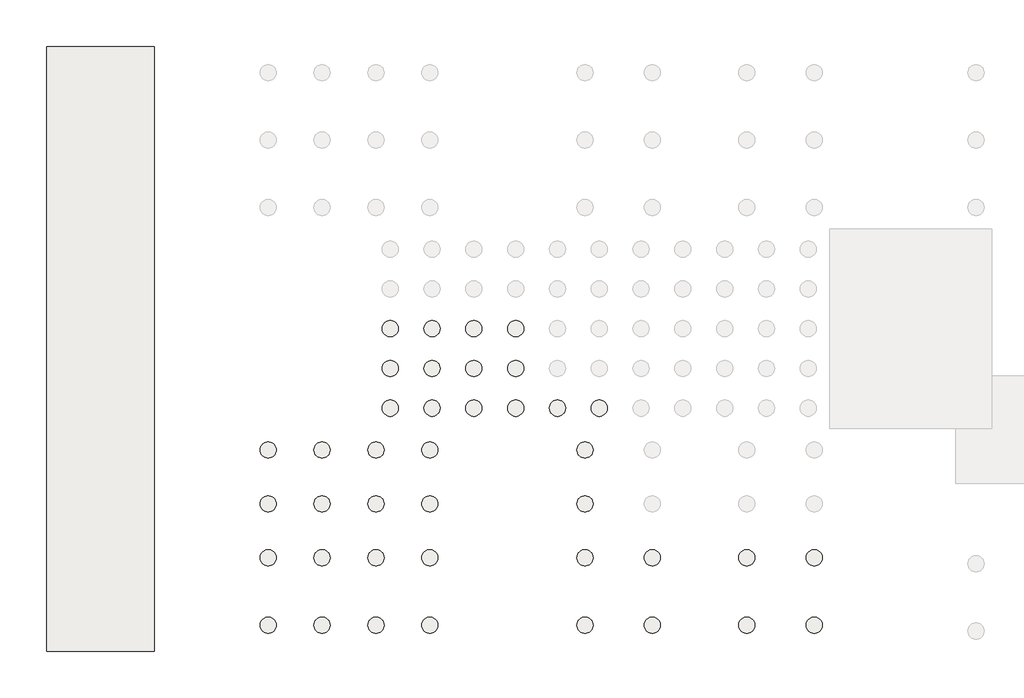
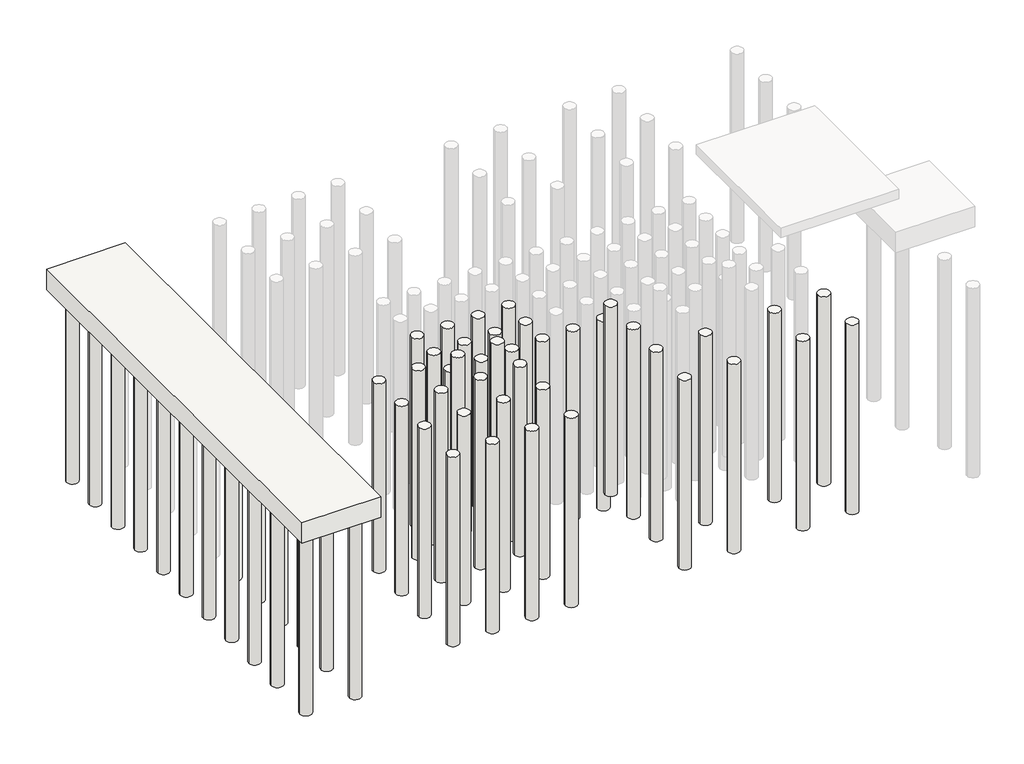
# One storey, part 1 of 3: 58 slabs.
"""IFC4 building model written with IfcOpenShell, lengths in millimetres."""

from ifc_helpers import new_model, si_unit, point, frame, frame_2d, origin, place, context, project, spatial, polyline, circle_curve, trimmed, segment, composite_curve, outline, extrude, element, save

model = new_model("IFC4")

# Units and contexts
model_context = context("Model", 3, world=origin())
ifc_project = project(units=[si_unit("LENGTHUNIT", "METRE", prefix="MILLI")], contexts=[model_context])

# Site, building, storey
site = spatial("IfcSite", under=ifc_project)
building = spatial("IfcBuilding", under=site)
storey = spatial("IfcBuildingStorey", under=building, Name="B.O.F(FDN)", Elevation=-2500.0279945)

# Slabs
placement = place(None, origin())
element("IfcSlab", 1, ObjectType="Foundation Rectangular(Non-Pile) : H_SF_ACF_W4000xL22440xT1100_Protection", at=placement, inside=storey, context=model_context, shape_type="SweptSolid", body=[
    extrude(outline(polyline([(1785.0, 41219.5208589), (1785.0, 18779.5208589), (-2215.0, 18779.5208589), (-2215.0, 41219.5208589), (1785.0, 41219.5208589)])), frame((0.0, 0.0, -3600.0279945), z_axis=(0.0, 0.0, 1.0), x_axis=(1.0, 0.0, 0.0)), (0.0, 0.0, 1.0), 1100.0),
])
element("IfcSlab", 2, ObjectType="Pile : H_SF_API_Steel Pile D508x12t_L10m", at=placement, inside=storey, context=model_context, shape_type="SweptSolid", body=[
    extrude(outline(composite_curve([segment(trimmed(circle_curve(frame_2d((-1465.0, 40249.5208589)), 300.0), [point((-1765.0, 40249.5208589))], [point((-1165.0, 40249.5208589))], False, "CARTESIAN"), True, "CONTINUOUS"), segment(trimmed(circle_curve(frame_2d((-1465.0, 40249.5208589)), 300.0), [point((-1165.0, 40249.5208589))], [point((-1765.0, 40249.5208589))], False, "CARTESIAN"), True, "CONTINUOUS")], self_intersect=False)), frame((0.0, 0.0, -13500.0279945), z_axis=(0.0, 0.0, 1.0), x_axis=(1.0, 0.0, 0.0)), (0.0, 0.0, 1.0), 10150.0),
])
element("IfcSlab", 3, ObjectType="Pile : H_SF_API_Steel Pile D508x12t_L10m", at=placement, inside=storey, context=model_context, shape_type="SweptSolid", body=[
    extrude(outline(composite_curve([segment(trimmed(circle_curve(frame_2d((-1465.0, 19749.5208589)), 300.0), [point((-1765.0, 19749.5208589))], [point((-1165.0, 19749.5208589))], False, "CARTESIAN"), True, "CONTINUOUS"), segment(trimmed(circle_curve(frame_2d((-1465.0, 19749.5208589)), 300.0), [point((-1165.0, 19749.5208589))], [point((-1765.0, 19749.5208589))], False, "CARTESIAN"), True, "CONTINUOUS")], self_intersect=False)), frame((0.0, 0.0, -13500.0279945), z_axis=(0.0, 0.0, 1.0), x_axis=(1.0, 0.0, 0.0)), (0.0, 0.0, 1.0), 10150.0),
])
element("IfcSlab", 4, ObjectType="Pile : H_SF_API_Steel Pile D508x12t_L10m", at=placement, inside=storey, context=model_context, shape_type="SweptSolid", body=[
    extrude(outline(composite_curve([segment(trimmed(circle_curve(frame_2d((1035.0, 19749.5208589)), 300.0), [point((1335.0, 19749.5208589))], [point((735.0, 19749.5208589))], False, "CARTESIAN"), True, "CONTINUOUS"), segment(trimmed(circle_curve(frame_2d((1035.0, 19749.5208589)), 300.0), [point((735.0, 19749.5208589))], [point((1335.0, 19749.5208589))], False, "CARTESIAN"), True, "CONTINUOUS")], self_intersect=False)), frame((0.0, 0.0, -13500.0279945), z_axis=(0.0, 0.0, 1.0), x_axis=(1.0, 0.0, 0.0)), (0.0, 0.0, 1.0), 10150.0),
])
element("IfcSlab", 5, ObjectType="Pile : H_SF_API_Steel Pile D508x12t_L10m", at=placement, inside=storey, context=model_context, shape_type="SweptSolid", body=[
    extrude(outline(composite_curve([segment(trimmed(circle_curve(frame_2d((-1465.0, 38249.5208589)), 300.0), [point((-1765.0, 38249.5208589))], [point((-1165.0, 38249.5208589))], False, "CARTESIAN"), True, "CONTINUOUS"), segment(trimmed(circle_curve(frame_2d((-1465.0, 38249.5208589)), 300.0), [point((-1165.0, 38249.5208589))], [point((-1765.0, 38249.5208589))], False, "CARTESIAN"), True, "CONTINUOUS")], self_intersect=False)), frame((0.0, 0.0, -13500.0279945), z_axis=(0.0, 0.0, 1.0), x_axis=(1.0, 0.0, 0.0)), (0.0, 0.0, 1.0), 10150.0),
])
element("IfcSlab", 6, ObjectType="Pile : H_SF_API_Steel Pile D508x12t_L10m", at=placement, inside=storey, context=model_context, shape_type="SweptSolid", body=[
    extrude(outline(composite_curve([segment(trimmed(circle_curve(frame_2d((-1465.0, 36249.5208589)), 300.0), [point((-1765.0, 36249.5208589))], [point((-1165.0, 36249.5208589))], False, "CARTESIAN"), True, "CONTINUOUS"), segment(trimmed(circle_curve(frame_2d((-1465.0, 36249.5208589)), 300.0), [point((-1165.0, 36249.5208589))], [point((-1765.0, 36249.5208589))], False, "CARTESIAN"), True, "CONTINUOUS")], self_intersect=False)), frame((0.0, 0.0, -13500.0279945), z_axis=(0.0, 0.0, 1.0), x_axis=(1.0, 0.0, 0.0)), (0.0, 0.0, 1.0), 10150.0),
])
element("IfcSlab", 7, ObjectType="Pile : H_SF_API_Steel Pile D508x12t_L10m", at=placement, inside=storey, context=model_context, shape_type="SweptSolid", body=[
    extrude(outline(composite_curve([segment(trimmed(circle_curve(frame_2d((-1465.0, 34249.5208589)), 300.0), [point((-1765.0, 34249.5208589))], [point((-1165.0, 34249.5208589))], False, "CARTESIAN"), True, "CONTINUOUS"), segment(trimmed(circle_curve(frame_2d((-1465.0, 34249.5208589)), 300.0), [point((-1165.0, 34249.5208589))], [point((-1765.0, 34249.5208589))], False, "CARTESIAN"), True, "CONTINUOUS")], self_intersect=False)), frame((0.0, 0.0, -13500.0279945), z_axis=(0.0, 0.0, 1.0), x_axis=(1.0, 0.0, 0.0)), (0.0, 0.0, 1.0), 10150.0),
])
element("IfcSlab", 8, ObjectType="Pile : H_SF_API_Steel Pile D508x12t_L10m", at=placement, inside=storey, context=model_context, shape_type="SweptSolid", body=[
    extrude(outline(composite_curve([segment(trimmed(circle_curve(frame_2d((-1465.0, 32249.5208589)), 300.0), [point((-1765.0, 32249.5208589))], [point((-1165.0, 32249.5208589))], False, "CARTESIAN"), True, "CONTINUOUS"), segment(trimmed(circle_curve(frame_2d((-1465.0, 32249.5208589)), 300.0), [point((-1165.0, 32249.5208589))], [point((-1765.0, 32249.5208589))], False, "CARTESIAN"), True, "CONTINUOUS")], self_intersect=False)), frame((0.0, 0.0, -13500.0279945), z_axis=(0.0, 0.0, 1.0), x_axis=(1.0, 0.0, 0.0)), (0.0, 0.0, 1.0), 10150.0),
])
element("IfcSlab", 9, ObjectType="Pile : H_SF_API_Steel Pile D508x12t_L10m", at=placement, inside=storey, context=model_context, shape_type="SweptSolid", body=[
    extrude(outline(composite_curve([segment(trimmed(circle_curve(frame_2d((-1465.0, 30249.5208589)), 300.0), [point((-1765.0, 30249.5208589))], [point((-1165.0, 30249.5208589))], False, "CARTESIAN"), True, "CONTINUOUS"), segment(trimmed(circle_curve(frame_2d((-1465.0, 30249.5208589)), 300.0), [point((-1165.0, 30249.5208589))], [point((-1765.0, 30249.5208589))], False, "CARTESIAN"), True, "CONTINUOUS")], self_intersect=False)), frame((0.0, 0.0, -13500.0279945), z_axis=(0.0, 0.0, 1.0), x_axis=(1.0, 0.0, 0.0)), (0.0, 0.0, 1.0), 10150.0),
])
element("IfcSlab", 10, ObjectType="Pile : H_SF_API_Steel Pile D508x12t_L10m", at=placement, inside=storey, context=model_context, shape_type="SweptSolid", body=[
    extrude(outline(composite_curve([segment(trimmed(circle_curve(frame_2d((1035.0, 30249.5208589)), 300.0), [point((1335.0, 30249.5208589))], [point((735.0, 30249.5208589))], False, "CARTESIAN"), True, "CONTINUOUS"), segment(trimmed(circle_curve(frame_2d((1035.0, 30249.5208589)), 300.0), [point((735.0, 30249.5208589))], [point((1335.0, 30249.5208589))], False, "CARTESIAN"), True, "CONTINUOUS")], self_intersect=False)), frame((0.0, 0.0, -13500.0279945), z_axis=(0.0, 0.0, 1.0), x_axis=(1.0, 0.0, 0.0)), (0.0, 0.0, 1.0), 10150.0),
])
element("IfcSlab", 11, ObjectType="Pile : H_SF_API_Steel Pile D508x12t_L10m", at=placement, inside=storey, context=model_context, shape_type="SweptSolid", body=[
    extrude(outline(composite_curve([segment(trimmed(circle_curve(frame_2d((-1465.0, 28249.5208589)), 300.0), [point((-1765.0, 28249.5208589))], [point((-1165.0, 28249.5208589))], False, "CARTESIAN"), True, "CONTINUOUS"), segment(trimmed(circle_curve(frame_2d((-1465.0, 28249.5208589)), 300.0), [point((-1165.0, 28249.5208589))], [point((-1765.0, 28249.5208589))], False, "CARTESIAN"), True, "CONTINUOUS")], self_intersect=False)), frame((0.0, 0.0, -13500.0279945), z_axis=(0.0, 0.0, 1.0), x_axis=(1.0, 0.0, 0.0)), (0.0, 0.0, 1.0), 10150.0),
])
element("IfcSlab", 12, ObjectType="Pile : H_SF_API_Steel Pile D508x12t_L10m", at=placement, inside=storey, context=model_context, shape_type="SweptSolid", body=[
    extrude(outline(composite_curve([segment(trimmed(circle_curve(frame_2d((1035.0, 28249.5208589)), 300.0), [point((1335.0, 28249.5208589))], [point((735.0, 28249.5208589))], False, "CARTESIAN"), True, "CONTINUOUS"), segment(trimmed(circle_curve(frame_2d((1035.0, 28249.5208589)), 300.0), [point((735.0, 28249.5208589))], [point((1335.0, 28249.5208589))], False, "CARTESIAN"), True, "CONTINUOUS")], self_intersect=False)), frame((0.0, 0.0, -13500.0279945), z_axis=(0.0, 0.0, 1.0), x_axis=(1.0, 0.0, 0.0)), (0.0, 0.0, 1.0), 10150.0),
])
element("IfcSlab", 13, ObjectType="Pile : H_SF_API_Steel Pile D508x12t_L10m", at=placement, inside=storey, context=model_context, shape_type="SweptSolid", body=[
    extrude(outline(composite_curve([segment(trimmed(circle_curve(frame_2d((-1465.0, 26249.5208589)), 300.0), [point((-1765.0, 26249.5208589))], [point((-1165.0, 26249.5208589))], False, "CARTESIAN"), True, "CONTINUOUS"), segment(trimmed(circle_curve(frame_2d((-1465.0, 26249.5208589)), 300.0), [point((-1165.0, 26249.5208589))], [point((-1765.0, 26249.5208589))], False, "CARTESIAN"), True, "CONTINUOUS")], self_intersect=False)), frame((0.0, 0.0, -13500.0279945), z_axis=(0.0, 0.0, 1.0), x_axis=(1.0, 0.0, 0.0)), (0.0, 0.0, 1.0), 10150.0),
])
element("IfcSlab", 14, ObjectType="Pile : H_SF_API_Steel Pile D508x12t_L10m", at=placement, inside=storey, context=model_context, shape_type="SweptSolid", body=[
    extrude(outline(composite_curve([segment(trimmed(circle_curve(frame_2d((1035.0, 26249.5208589)), 300.0), [point((1335.0, 26249.5208589))], [point((735.0, 26249.5208589))], False, "CARTESIAN"), True, "CONTINUOUS"), segment(trimmed(circle_curve(frame_2d((1035.0, 26249.5208589)), 300.0), [point((735.0, 26249.5208589))], [point((1335.0, 26249.5208589))], False, "CARTESIAN"), True, "CONTINUOUS")], self_intersect=False)), frame((0.0, 0.0, -13500.0279945), z_axis=(0.0, 0.0, 1.0), x_axis=(1.0, 0.0, 0.0)), (0.0, 0.0, 1.0), 10150.0),
])
element("IfcSlab", 15, ObjectType="Pile : H_SF_API_Steel Pile D508x12t_L10m", at=placement, inside=storey, context=model_context, shape_type="SweptSolid", body=[
    extrude(outline(composite_curve([segment(trimmed(circle_curve(frame_2d((-1465.0, 24249.5208589)), 300.0), [point((-1765.0, 24249.5208589))], [point((-1165.0, 24249.5208589))], False, "CARTESIAN"), True, "CONTINUOUS"), segment(trimmed(circle_curve(frame_2d((-1465.0, 24249.5208589)), 300.0), [point((-1165.0, 24249.5208589))], [point((-1765.0, 24249.5208589))], False, "CARTESIAN"), True, "CONTINUOUS")], self_intersect=False)), frame((0.0, 0.0, -13500.0279945), z_axis=(0.0, 0.0, 1.0), x_axis=(1.0, 0.0, 0.0)), (0.0, 0.0, 1.0), 10150.0),
])
element("IfcSlab", 16, ObjectType="Pile : H_SF_API_Steel Pile D508x12t_L10m", at=placement, inside=storey, context=model_context, shape_type="SweptSolid", body=[
    extrude(outline(composite_curve([segment(trimmed(circle_curve(frame_2d((1035.0, 24249.5208589)), 300.0), [point((1335.0, 24249.5208589))], [point((735.0, 24249.5208589))], False, "CARTESIAN"), True, "CONTINUOUS"), segment(trimmed(circle_curve(frame_2d((1035.0, 24249.5208589)), 300.0), [point((735.0, 24249.5208589))], [point((1335.0, 24249.5208589))], False, "CARTESIAN"), True, "CONTINUOUS")], self_intersect=False)), frame((0.0, 0.0, -13500.0279945), z_axis=(0.0, 0.0, 1.0), x_axis=(1.0, 0.0, 0.0)), (0.0, 0.0, 1.0), 10150.0),
])
element("IfcSlab", 17, ObjectType="Pile : H_SF_API_Steel Pile D508x12t_L10m", at=placement, inside=storey, context=model_context, shape_type="SweptSolid", body=[
    extrude(outline(composite_curve([segment(trimmed(circle_curve(frame_2d((-1465.0, 22249.5208589)), 300.0), [point((-1765.0, 22249.5208589))], [point((-1165.0, 22249.5208589))], False, "CARTESIAN"), True, "CONTINUOUS"), segment(trimmed(circle_curve(frame_2d((-1465.0, 22249.5208589)), 300.0), [point((-1165.0, 22249.5208589))], [point((-1765.0, 22249.5208589))], False, "CARTESIAN"), True, "CONTINUOUS")], self_intersect=False)), frame((0.0, 0.0, -13500.0279945), z_axis=(0.0, 0.0, 1.0), x_axis=(1.0, 0.0, 0.0)), (0.0, 0.0, 1.0), 10150.0),
])
element("IfcSlab", 18, ObjectType="Pile : H_SF_API_Steel Pile D508x12t_L10m", at=placement, inside=storey, context=model_context, shape_type="SweptSolid", body=[
    extrude(outline(composite_curve([segment(trimmed(circle_curve(frame_2d((1035.0, 22249.5208589)), 300.0), [point((1335.0, 22249.5208589))], [point((735.0, 22249.5208589))], False, "CARTESIAN"), True, "CONTINUOUS"), segment(trimmed(circle_curve(frame_2d((1035.0, 22249.5208589)), 300.0), [point((735.0, 22249.5208589))], [point((1335.0, 22249.5208589))], False, "CARTESIAN"), True, "CONTINUOUS")], self_intersect=False)), frame((0.0, 0.0, -13500.0279945), z_axis=(0.0, 0.0, 1.0), x_axis=(1.0, 0.0, 0.0)), (0.0, 0.0, 1.0), 10150.0),
])
element("IfcSlab", 19, ObjectType="Pile : H_SF_API_Steel Pile D508x12t_L10m", at=placement, inside=storey, context=model_context, shape_type="SweptSolid", body=[
    extrude(outline(composite_curve([segment(trimmed(circle_curve(frame_2d((8000.0, 19749.5208589)), 300.0), [point((8300.0, 19749.5208589))], [point((7700.0, 19749.5208589))], False, "CARTESIAN"), True, "CONTINUOUS"), segment(trimmed(circle_curve(frame_2d((8000.0, 19749.5208589)), 300.0), [point((7700.0, 19749.5208589))], [point((8300.0, 19749.5208589))], False, "CARTESIAN"), True, "CONTINUOUS")], self_intersect=False)), frame((0.0, 0.0, -12400.0279945), z_axis=(0.0, 0.0, 1.0), x_axis=(1.0, 0.0, 0.0)), (0.0, 0.0, 1.0), 10150.0),
])
element("IfcSlab", 20, ObjectType="Pile : H_SF_API_Steel Pile D508x12t_L10m", at=placement, inside=storey, context=model_context, shape_type="SweptSolid", body=[
    extrude(outline(composite_curve([segment(trimmed(circle_curve(frame_2d((6000.0, 19749.5208589)), 300.0), [point((5700.0, 19749.5208589))], [point((6300.0, 19749.5208589))], False, "CARTESIAN"), True, "CONTINUOUS"), segment(trimmed(circle_curve(frame_2d((6000.0, 19749.5208589)), 300.0), [point((6300.0, 19749.5208589))], [point((5700.0, 19749.5208589))], False, "CARTESIAN"), True, "CONTINUOUS")], self_intersect=False)), frame((0.0, 0.0, -12400.0279945), z_axis=(0.0, 0.0, 1.0), x_axis=(1.0, 0.0, 0.0)), (0.0, 0.0, 1.0), 10150.0),
])
element("IfcSlab", 21, ObjectType="Pile : H_SF_API_Steel Pile D508x12t_L10m", at=placement, inside=storey, context=model_context, shape_type="SweptSolid", body=[
    extrude(outline(composite_curve([segment(trimmed(circle_curve(frame_2d((8000.0, 22249.5208589)), 300.0), [point((8300.0, 22249.5208589))], [point((7700.0, 22249.5208589))], False, "CARTESIAN"), True, "CONTINUOUS"), segment(trimmed(circle_curve(frame_2d((8000.0, 22249.5208589)), 300.0), [point((7700.0, 22249.5208589))], [point((8300.0, 22249.5208589))], False, "CARTESIAN"), True, "CONTINUOUS")], self_intersect=False)), frame((0.0, 0.0, -12400.0279945), z_axis=(0.0, 0.0, 1.0), x_axis=(1.0, 0.0, 0.0)), (0.0, 0.0, 1.0), 10150.0),
])
element("IfcSlab", 22, ObjectType="Pile : H_SF_API_Steel Pile D508x12t_L10m", at=placement, inside=storey, context=model_context, shape_type="SweptSolid", body=[
    extrude(outline(composite_curve([segment(trimmed(circle_curve(frame_2d((6000.0, 22249.5208589)), 300.0), [point((5700.0, 22249.5208589))], [point((6300.0, 22249.5208589))], False, "CARTESIAN"), True, "CONTINUOUS"), segment(trimmed(circle_curve(frame_2d((6000.0, 22249.5208589)), 300.0), [point((6300.0, 22249.5208589))], [point((5700.0, 22249.5208589))], False, "CARTESIAN"), True, "CONTINUOUS")], self_intersect=False)), frame((0.0, 0.0, -12400.0279945), z_axis=(0.0, 0.0, 1.0), x_axis=(1.0, 0.0, 0.0)), (0.0, 0.0, 1.0), 10150.0),
])
element("IfcSlab", 23, ObjectType="Pile : H_SF_API_Steel Pile D508x12t_L10m", at=placement, inside=storey, context=model_context, shape_type="SweptSolid", body=[
    extrude(outline(composite_curve([segment(trimmed(circle_curve(frame_2d((8000.0, 24249.5208589)), 300.0), [point((8300.0, 24249.5208589))], [point((7700.0, 24249.5208589))], False, "CARTESIAN"), True, "CONTINUOUS"), segment(trimmed(circle_curve(frame_2d((8000.0, 24249.5208589)), 300.0), [point((7700.0, 24249.5208589))], [point((8300.0, 24249.5208589))], False, "CARTESIAN"), True, "CONTINUOUS")], self_intersect=False)), frame((0.0, 0.0, -12400.0279945), z_axis=(0.0, 0.0, 1.0), x_axis=(1.0, 0.0, 0.0)), (0.0, 0.0, 1.0), 10150.0),
])
element("IfcSlab", 24, ObjectType="Pile : H_SF_API_Steel Pile D508x12t_L10m", at=placement, inside=storey, context=model_context, shape_type="SweptSolid", body=[
    extrude(outline(composite_curve([segment(trimmed(circle_curve(frame_2d((6000.0, 24249.5208589)), 300.0), [point((5700.0, 24249.5208589))], [point((6300.0, 24249.5208589))], False, "CARTESIAN"), True, "CONTINUOUS"), segment(trimmed(circle_curve(frame_2d((6000.0, 24249.5208589)), 300.0), [point((6300.0, 24249.5208589))], [point((5700.0, 24249.5208589))], False, "CARTESIAN"), True, "CONTINUOUS")], self_intersect=False)), frame((0.0, 0.0, -12400.0279945), z_axis=(0.0, 0.0, 1.0), x_axis=(1.0, 0.0, 0.0)), (0.0, 0.0, 1.0), 10150.0),
])
element("IfcSlab", 25, ObjectType="Pile : H_SF_API_Steel Pile D508x12t_L10m", at=placement, inside=storey, context=model_context, shape_type="SweptSolid", body=[
    extrude(outline(composite_curve([segment(trimmed(circle_curve(frame_2d((8000.0, 26249.5208589)), 300.0), [point((8300.0, 26249.5208589))], [point((7700.0, 26249.5208589))], False, "CARTESIAN"), True, "CONTINUOUS"), segment(trimmed(circle_curve(frame_2d((8000.0, 26249.5208589)), 300.0), [point((7700.0, 26249.5208589))], [point((8300.0, 26249.5208589))], False, "CARTESIAN"), True, "CONTINUOUS")], self_intersect=False)), frame((0.0, 0.0, -12400.0279945), z_axis=(0.0, 0.0, 1.0), x_axis=(1.0, 0.0, 0.0)), (0.0, 0.0, 1.0), 10150.0),
])
element("IfcSlab", 26, ObjectType="Pile : H_SF_API_Steel Pile D508x12t_L10m", at=placement, inside=storey, context=model_context, shape_type="SweptSolid", body=[
    extrude(outline(composite_curve([segment(trimmed(circle_curve(frame_2d((6000.0, 26249.5208589)), 300.0), [point((5700.0, 26249.5208589))], [point((6300.0, 26249.5208589))], False, "CARTESIAN"), True, "CONTINUOUS"), segment(trimmed(circle_curve(frame_2d((6000.0, 26249.5208589)), 300.0), [point((6300.0, 26249.5208589))], [point((5700.0, 26249.5208589))], False, "CARTESIAN"), True, "CONTINUOUS")], self_intersect=False)), frame((0.0, 0.0, -12400.0279945), z_axis=(0.0, 0.0, 1.0), x_axis=(1.0, 0.0, 0.0)), (0.0, 0.0, 1.0), 10150.0),
])
element("IfcSlab", 27, ObjectType="Pile : H_SF_API_Steel Pile D508x12t_L10m", at=placement, inside=storey, context=model_context, shape_type="SweptSolid", body=[
    extrude(outline(composite_curve([segment(trimmed(circle_curve(frame_2d((12000.0, 19749.5208589)), 300.0), [point((12300.0, 19749.5208589))], [point((11700.0, 19749.5208589))], False, "CARTESIAN"), True, "CONTINUOUS"), segment(trimmed(circle_curve(frame_2d((12000.0, 19749.5208589)), 300.0), [point((11700.0, 19749.5208589))], [point((12300.0, 19749.5208589))], False, "CARTESIAN"), True, "CONTINUOUS")], self_intersect=False)), frame((0.0, 0.0, -12400.0279945), z_axis=(0.0, 0.0, 1.0), x_axis=(1.0, 0.0, 0.0)), (0.0, 0.0, 1.0), 10150.0),
])
element("IfcSlab", 28, ObjectType="Pile : H_SF_API_Steel Pile D508x12t_L10m", at=placement, inside=storey, context=model_context, shape_type="SweptSolid", body=[
    extrude(outline(composite_curve([segment(trimmed(circle_curve(frame_2d((10000.0, 19749.5208589)), 300.0), [point((9700.0, 19749.5208589))], [point((10300.0, 19749.5208589))], False, "CARTESIAN"), True, "CONTINUOUS"), segment(trimmed(circle_curve(frame_2d((10000.0, 19749.5208589)), 300.0), [point((10300.0, 19749.5208589))], [point((9700.0, 19749.5208589))], False, "CARTESIAN"), True, "CONTINUOUS")], self_intersect=False)), frame((0.0, 0.0, -12400.0279945), z_axis=(0.0, 0.0, 1.0), x_axis=(1.0, 0.0, 0.0)), (0.0, 0.0, 1.0), 10150.0),
])
element("IfcSlab", 29, ObjectType="Pile : H_SF_API_Steel Pile D508x12t_L10m", at=placement, inside=storey, context=model_context, shape_type="SweptSolid", body=[
    extrude(outline(composite_curve([segment(trimmed(circle_curve(frame_2d((12000.0, 22249.5208589)), 300.0), [point((12300.0, 22249.5208589))], [point((11700.0, 22249.5208589))], False, "CARTESIAN"), True, "CONTINUOUS"), segment(trimmed(circle_curve(frame_2d((12000.0, 22249.5208589)), 300.0), [point((11700.0, 22249.5208589))], [point((12300.0, 22249.5208589))], False, "CARTESIAN"), True, "CONTINUOUS")], self_intersect=False)), frame((0.0, 0.0, -12400.0279945), z_axis=(0.0, 0.0, 1.0), x_axis=(1.0, 0.0, 0.0)), (0.0, 0.0, 1.0), 10150.0),
])
element("IfcSlab", 30, ObjectType="Pile : H_SF_API_Steel Pile D508x12t_L10m", at=placement, inside=storey, context=model_context, shape_type="SweptSolid", body=[
    extrude(outline(composite_curve([segment(trimmed(circle_curve(frame_2d((10000.0, 22249.5208589)), 300.0), [point((9700.0, 22249.5208589))], [point((10300.0, 22249.5208589))], False, "CARTESIAN"), True, "CONTINUOUS"), segment(trimmed(circle_curve(frame_2d((10000.0, 22249.5208589)), 300.0), [point((10300.0, 22249.5208589))], [point((9700.0, 22249.5208589))], False, "CARTESIAN"), True, "CONTINUOUS")], self_intersect=False)), frame((0.0, 0.0, -12400.0279945), z_axis=(0.0, 0.0, 1.0), x_axis=(1.0, 0.0, 0.0)), (0.0, 0.0, 1.0), 10150.0),
])
element("IfcSlab", 31, ObjectType="Pile : H_SF_API_Steel Pile D508x12t_L10m", at=placement, inside=storey, context=model_context, shape_type="SweptSolid", body=[
    extrude(outline(composite_curve([segment(trimmed(circle_curve(frame_2d((12000.0, 24249.5208589)), 300.0), [point((12300.0, 24249.5208589))], [point((11700.0, 24249.5208589))], False, "CARTESIAN"), True, "CONTINUOUS"), segment(trimmed(circle_curve(frame_2d((12000.0, 24249.5208589)), 300.0), [point((11700.0, 24249.5208589))], [point((12300.0, 24249.5208589))], False, "CARTESIAN"), True, "CONTINUOUS")], self_intersect=False)), frame((0.0, 0.0, -12400.0279945), z_axis=(0.0, 0.0, 1.0), x_axis=(1.0, 0.0, 0.0)), (0.0, 0.0, 1.0), 10150.0),
])
element("IfcSlab", 32, ObjectType="Pile : H_SF_API_Steel Pile D508x12t_L10m", at=placement, inside=storey, context=model_context, shape_type="SweptSolid", body=[
    extrude(outline(composite_curve([segment(trimmed(circle_curve(frame_2d((10000.0, 24249.5208589)), 300.0), [point((9700.0, 24249.5208589))], [point((10300.0, 24249.5208589))], False, "CARTESIAN"), True, "CONTINUOUS"), segment(trimmed(circle_curve(frame_2d((10000.0, 24249.5208589)), 300.0), [point((10300.0, 24249.5208589))], [point((9700.0, 24249.5208589))], False, "CARTESIAN"), True, "CONTINUOUS")], self_intersect=False)), frame((0.0, 0.0, -12400.0279945), z_axis=(0.0, 0.0, 1.0), x_axis=(1.0, 0.0, 0.0)), (0.0, 0.0, 1.0), 10150.0),
])
element("IfcSlab", 33, ObjectType="Pile : H_SF_API_Steel Pile D508x12t_L10m", at=placement, inside=storey, context=model_context, shape_type="SweptSolid", body=[
    extrude(outline(composite_curve([segment(trimmed(circle_curve(frame_2d((12000.0, 26249.5208589)), 300.0), [point((12300.0, 26249.5208589))], [point((11700.0, 26249.5208589))], False, "CARTESIAN"), True, "CONTINUOUS"), segment(trimmed(circle_curve(frame_2d((12000.0, 26249.5208589)), 300.0), [point((11700.0, 26249.5208589))], [point((12300.0, 26249.5208589))], False, "CARTESIAN"), True, "CONTINUOUS")], self_intersect=False)), frame((0.0, 0.0, -12400.0279945), z_axis=(0.0, 0.0, 1.0), x_axis=(1.0, 0.0, 0.0)), (0.0, 0.0, 1.0), 10150.0),
])
element("IfcSlab", 34, ObjectType="Pile : H_SF_API_Steel Pile D508x12t_L10m", at=placement, inside=storey, context=model_context, shape_type="SweptSolid", body=[
    extrude(outline(composite_curve([segment(trimmed(circle_curve(frame_2d((10000.0, 26249.5208589)), 300.0), [point((9700.0, 26249.5208589))], [point((10300.0, 26249.5208589))], False, "CARTESIAN"), True, "CONTINUOUS"), segment(trimmed(circle_curve(frame_2d((10000.0, 26249.5208589)), 300.0), [point((10300.0, 26249.5208589))], [point((9700.0, 26249.5208589))], False, "CARTESIAN"), True, "CONTINUOUS")], self_intersect=False)), frame((0.0, 0.0, -12400.0279945), z_axis=(0.0, 0.0, 1.0), x_axis=(1.0, 0.0, 0.0)), (0.0, 0.0, 1.0), 10150.0),
])
element("IfcSlab", 35, ObjectType="Pile : H_SF_API_Steel Pile D508x12t_L10m", at=placement, inside=storey, context=model_context, shape_type="SweptSolid", body=[
    extrude(outline(composite_curve([segment(trimmed(circle_curve(frame_2d((20250.0, 19749.5208589)), 300.0), [point((20550.0, 19749.5208589))], [point((19950.0, 19749.5208589))], False, "CARTESIAN"), True, "CONTINUOUS"), segment(trimmed(circle_curve(frame_2d((20250.0, 19749.5208589)), 300.0), [point((19950.0, 19749.5208589))], [point((20550.0, 19749.5208589))], False, "CARTESIAN"), True, "CONTINUOUS")], self_intersect=False)), frame((0.0, 0.0, -12400.0279945), z_axis=(0.0, 0.0, 1.0), x_axis=(1.0, 0.0, 0.0)), (0.0, 0.0, 1.0), 10150.0),
])
element("IfcSlab", 36, ObjectType="Pile : H_SF_API_Steel Pile D508x12t_L10m", at=placement, inside=storey, context=model_context, shape_type="SweptSolid", body=[
    extrude(outline(composite_curve([segment(trimmed(circle_curve(frame_2d((17750.0, 19749.5208589)), 300.0), [point((17450.0, 19749.5208589))], [point((18050.0, 19749.5208589))], False, "CARTESIAN"), True, "CONTINUOUS"), segment(trimmed(circle_curve(frame_2d((17750.0, 19749.5208589)), 300.0), [point((18050.0, 19749.5208589))], [point((17450.0, 19749.5208589))], False, "CARTESIAN"), True, "CONTINUOUS")], self_intersect=False)), frame((0.0, 0.0, -12400.0279945), z_axis=(0.0, 0.0, 1.0), x_axis=(1.0, 0.0, 0.0)), (0.0, 0.0, 1.0), 10150.0),
])
element("IfcSlab", 37, ObjectType="Pile : H_SF_API_Steel Pile D508x12t_L10m", at=placement, inside=storey, context=model_context, shape_type="SweptSolid", body=[
    extrude(outline(composite_curve([segment(trimmed(circle_curve(frame_2d((20250.0, 22249.5208589)), 300.0), [point((20550.0, 22249.5208589))], [point((19950.0, 22249.5208589))], False, "CARTESIAN"), True, "CONTINUOUS"), segment(trimmed(circle_curve(frame_2d((20250.0, 22249.5208589)), 300.0), [point((19950.0, 22249.5208589))], [point((20550.0, 22249.5208589))], False, "CARTESIAN"), True, "CONTINUOUS")], self_intersect=False)), frame((0.0, 0.0, -12400.0279945), z_axis=(0.0, 0.0, 1.0), x_axis=(1.0, 0.0, 0.0)), (0.0, 0.0, 1.0), 10150.0),
])
element("IfcSlab", 38, ObjectType="Pile : H_SF_API_Steel Pile D508x12t_L10m", at=placement, inside=storey, context=model_context, shape_type="SweptSolid", body=[
    extrude(outline(composite_curve([segment(trimmed(circle_curve(frame_2d((17750.0, 22249.5208589)), 300.0), [point((17450.0, 22249.5208589))], [point((18050.0, 22249.5208589))], False, "CARTESIAN"), True, "CONTINUOUS"), segment(trimmed(circle_curve(frame_2d((17750.0, 22249.5208589)), 300.0), [point((18050.0, 22249.5208589))], [point((17450.0, 22249.5208589))], False, "CARTESIAN"), True, "CONTINUOUS")], self_intersect=False)), frame((0.0, 0.0, -12400.0279945), z_axis=(0.0, 0.0, 1.0), x_axis=(1.0, 0.0, 0.0)), (0.0, 0.0, 1.0), 10150.0),
])
element("IfcSlab", 39, ObjectType="Pile : H_SF_API_Steel Pile D508x12t_L10m", at=placement, inside=storey, context=model_context, shape_type="SweptSolid", body=[
    extrude(outline(composite_curve([segment(trimmed(circle_curve(frame_2d((17750.0, 24249.5208589)), 300.0), [point((17450.0, 24249.5208589))], [point((18050.0, 24249.5208589))], False, "CARTESIAN"), True, "CONTINUOUS"), segment(trimmed(circle_curve(frame_2d((17750.0, 24249.5208589)), 300.0), [point((18050.0, 24249.5208589))], [point((17450.0, 24249.5208589))], False, "CARTESIAN"), True, "CONTINUOUS")], self_intersect=False)), frame((0.0, 0.0, -12400.0279945), z_axis=(0.0, 0.0, 1.0), x_axis=(1.0, 0.0, 0.0)), (0.0, 0.0, 1.0), 10150.0),
])
element("IfcSlab", 40, ObjectType="Pile : H_SF_API_Steel Pile D508x12t_L10m", at=placement, inside=storey, context=model_context, shape_type="SweptSolid", body=[
    extrude(outline(composite_curve([segment(trimmed(circle_curve(frame_2d((17750.0, 26249.5208589)), 300.0), [point((17450.0, 26249.5208589))], [point((18050.0, 26249.5208589))], False, "CARTESIAN"), True, "CONTINUOUS"), segment(trimmed(circle_curve(frame_2d((17750.0, 26249.5208589)), 300.0), [point((18050.0, 26249.5208589))], [point((17450.0, 26249.5208589))], False, "CARTESIAN"), True, "CONTINUOUS")], self_intersect=False)), frame((0.0, 0.0, -12400.0279945), z_axis=(0.0, 0.0, 1.0), x_axis=(1.0, 0.0, 0.0)), (0.0, 0.0, 1.0), 10150.0),
])
element("IfcSlab", 41, ObjectType="Pile : H_SF_API_Steel Pile D508x12t_L10m", at=placement, inside=storey, context=model_context, shape_type="SweptSolid", body=[
    extrude(outline(composite_curve([segment(trimmed(circle_curve(frame_2d((26250.0, 19749.5208589)), 300.0), [point((26550.0, 19749.5208589))], [point((25950.0, 19749.5208589))], False, "CARTESIAN"), True, "CONTINUOUS"), segment(trimmed(circle_curve(frame_2d((26250.0, 19749.5208589)), 300.0), [point((25950.0, 19749.5208589))], [point((26550.0, 19749.5208589))], False, "CARTESIAN"), True, "CONTINUOUS")], self_intersect=False)), frame((0.0, 0.0, -12400.0279945), z_axis=(0.0, 0.0, 1.0), x_axis=(1.0, 0.0, 0.0)), (0.0, 0.0, 1.0), 10150.0),
])
element("IfcSlab", 42, ObjectType="Pile : H_SF_API_Steel Pile D508x12t_L10m", at=placement, inside=storey, context=model_context, shape_type="SweptSolid", body=[
    extrude(outline(composite_curve([segment(trimmed(circle_curve(frame_2d((23750.0, 19749.5208589)), 300.0), [point((23450.0, 19749.5208589))], [point((24050.0, 19749.5208589))], False, "CARTESIAN"), True, "CONTINUOUS"), segment(trimmed(circle_curve(frame_2d((23750.0, 19749.5208589)), 300.0), [point((24050.0, 19749.5208589))], [point((23450.0, 19749.5208589))], False, "CARTESIAN"), True, "CONTINUOUS")], self_intersect=False)), frame((0.0, 0.0, -12400.0279945), z_axis=(0.0, 0.0, 1.0), x_axis=(1.0, 0.0, 0.0)), (0.0, 0.0, 1.0), 10150.0),
])
element("IfcSlab", 43, ObjectType="Pile : H_SF_API_Steel Pile D508x12t_L10m", at=placement, inside=storey, context=model_context, shape_type="SweptSolid", body=[
    extrude(outline(composite_curve([segment(trimmed(circle_curve(frame_2d((26250.0, 22249.5208589)), 300.0), [point((26550.0, 22249.5208589))], [point((25950.0, 22249.5208589))], False, "CARTESIAN"), True, "CONTINUOUS"), segment(trimmed(circle_curve(frame_2d((26250.0, 22249.5208589)), 300.0), [point((25950.0, 22249.5208589))], [point((26550.0, 22249.5208589))], False, "CARTESIAN"), True, "CONTINUOUS")], self_intersect=False)), frame((0.0, 0.0, -12400.0279945), z_axis=(0.0, 0.0, 1.0), x_axis=(1.0, 0.0, 0.0)), (0.0, 0.0, 1.0), 10150.0),
])
element("IfcSlab", 44, ObjectType="Pile : H_SF_API_Steel Pile D508x12t_L10m", at=placement, inside=storey, context=model_context, shape_type="SweptSolid", body=[
    extrude(outline(composite_curve([segment(trimmed(circle_curve(frame_2d((23750.0, 22249.5208589)), 300.0), [point((23450.0, 22249.5208589))], [point((24050.0, 22249.5208589))], False, "CARTESIAN"), True, "CONTINUOUS"), segment(trimmed(circle_curve(frame_2d((23750.0, 22249.5208589)), 300.0), [point((24050.0, 22249.5208589))], [point((23450.0, 22249.5208589))], False, "CARTESIAN"), True, "CONTINUOUS")], self_intersect=False)), frame((0.0, 0.0, -12400.0279945), z_axis=(0.0, 0.0, 1.0), x_axis=(1.0, 0.0, 0.0)), (0.0, 0.0, 1.0), 10150.0),
])
element("IfcSlab", 45, ObjectType="Pile : H_SF_API_Steel Pile D508x12t_L10m", at=placement, inside=storey, context=model_context, shape_type="SweptSolid", body=[
    extrude(outline(composite_curve([segment(trimmed(circle_curve(frame_2d((10530.0, 27799.5208589)), 300.0), [point((10230.0, 27799.5208589))], [point((10830.0, 27799.5208589))], False, "CARTESIAN"), True, "CONTINUOUS"), segment(trimmed(circle_curve(frame_2d((10530.0, 27799.5208589)), 300.0), [point((10830.0, 27799.5208589))], [point((10230.0, 27799.5208589))], False, "CARTESIAN"), True, "CONTINUOUS")], self_intersect=False)), frame((0.0, 0.0, -14300.0279945), z_axis=(0.0, 0.0, 1.0), x_axis=(1.0, 0.0, 0.0)), (0.0, 0.0, 1.0), 10150.0),
])
element("IfcSlab", 46, ObjectType="Pile : H_SF_API_Steel Pile D508x12t_L10m", at=placement, inside=storey, context=model_context, shape_type="SweptSolid", body=[
    extrude(outline(composite_curve([segment(trimmed(circle_curve(frame_2d((10530.0, 29274.5208589)), 300.0), [point((10230.0, 29274.5208589))], [point((10830.0, 29274.5208589))], False, "CARTESIAN"), True, "CONTINUOUS"), segment(trimmed(circle_curve(frame_2d((10530.0, 29274.5208589)), 300.0), [point((10830.0, 29274.5208589))], [point((10230.0, 29274.5208589))], False, "CARTESIAN"), True, "CONTINUOUS")], self_intersect=False)), frame((0.0, 0.0, -14300.0279945), z_axis=(0.0, 0.0, 1.0), x_axis=(1.0, 0.0, 0.0)), (0.0, 0.0, 1.0), 10150.0),
])
element("IfcSlab", 47, ObjectType="Pile : H_SF_API_Steel Pile D508x12t_L10m", at=placement, inside=storey, context=model_context, shape_type="SweptSolid", body=[
    extrude(outline(composite_curve([segment(trimmed(circle_curve(frame_2d((10530.0, 30749.5208589)), 300.0), [point((10230.0, 30749.5208589))], [point((10830.0, 30749.5208589))], False, "CARTESIAN"), True, "CONTINUOUS"), segment(trimmed(circle_curve(frame_2d((10530.0, 30749.5208589)), 300.0), [point((10830.0, 30749.5208589))], [point((10230.0, 30749.5208589))], False, "CARTESIAN"), True, "CONTINUOUS")], self_intersect=False)), frame((0.0, 0.0, -14300.0279945), z_axis=(0.0, 0.0, 1.0), x_axis=(1.0, 0.0, 0.0)), (0.0, 0.0, 1.0), 10150.0),
])
element("IfcSlab", 48, ObjectType="Pile : H_SF_API_Steel Pile D508x12t_L10m", at=placement, inside=storey, context=model_context, shape_type="SweptSolid", body=[
    extrude(outline(composite_curve([segment(trimmed(circle_curve(frame_2d((18280.0, 27799.5208589)), 300.0), [point((18580.0, 27799.5208589))], [point((17980.0, 27799.5208589))], False, "CARTESIAN"), True, "CONTINUOUS"), segment(trimmed(circle_curve(frame_2d((18280.0, 27799.5208589)), 300.0), [point((17980.0, 27799.5208589))], [point((18580.0, 27799.5208589))], False, "CARTESIAN"), True, "CONTINUOUS")], self_intersect=False)), frame((0.0, 0.0, -14300.0279945), z_axis=(0.0, 0.0, 1.0), x_axis=(1.0, 0.0, 0.0)), (0.0, 0.0, 1.0), 10150.0),
])
element("IfcSlab", 49, ObjectType="Pile : H_SF_API_Steel Pile D508x12t_L10m", at=placement, inside=storey, context=model_context, shape_type="SweptSolid", body=[
    extrude(outline(composite_curve([segment(trimmed(circle_curve(frame_2d((16730.0, 27799.5208589)), 300.0), [point((17030.0, 27799.5208589))], [point((16430.0, 27799.5208589))], False, "CARTESIAN"), True, "CONTINUOUS"), segment(trimmed(circle_curve(frame_2d((16730.0, 27799.5208589)), 300.0), [point((16430.0, 27799.5208589))], [point((17030.0, 27799.5208589))], False, "CARTESIAN"), True, "CONTINUOUS")], self_intersect=False)), frame((0.0, 0.0, -14300.0279945), z_axis=(0.0, 0.0, 1.0), x_axis=(1.0, 0.0, 0.0)), (0.0, 0.0, 1.0), 10150.0),
])
element("IfcSlab", 50, ObjectType="Pile : H_SF_API_Steel Pile D508x12t_L10m", at=placement, inside=storey, context=model_context, shape_type="SweptSolid", body=[
    extrude(outline(composite_curve([segment(trimmed(circle_curve(frame_2d((15180.0, 27799.5208589)), 300.0), [point((15480.0, 27799.5208589))], [point((14880.0, 27799.5208589))], False, "CARTESIAN"), True, "CONTINUOUS"), segment(trimmed(circle_curve(frame_2d((15180.0, 27799.5208589)), 300.0), [point((14880.0, 27799.5208589))], [point((15480.0, 27799.5208589))], False, "CARTESIAN"), True, "CONTINUOUS")], self_intersect=False)), frame((0.0, 0.0, -14300.0279945), z_axis=(0.0, 0.0, 1.0), x_axis=(1.0, 0.0, 0.0)), (0.0, 0.0, 1.0), 10150.0),
])
element("IfcSlab", 51, ObjectType="Pile : H_SF_API_Steel Pile D508x12t_L10m", at=placement, inside=storey, context=model_context, shape_type="SweptSolid", body=[
    extrude(outline(composite_curve([segment(trimmed(circle_curve(frame_2d((15180.0, 29274.5208589)), 300.0), [point((15480.0, 29274.5208589))], [point((14880.0, 29274.5208589))], False, "CARTESIAN"), True, "CONTINUOUS"), segment(trimmed(circle_curve(frame_2d((15180.0, 29274.5208589)), 300.0), [point((14880.0, 29274.5208589))], [point((15480.0, 29274.5208589))], False, "CARTESIAN"), True, "CONTINUOUS")], self_intersect=False)), frame((0.0, 0.0, -14300.0279945), z_axis=(0.0, 0.0, 1.0), x_axis=(1.0, 0.0, 0.0)), (0.0, 0.0, 1.0), 10150.0),
])
element("IfcSlab", 52, ObjectType="Pile : H_SF_API_Steel Pile D508x12t_L10m", at=placement, inside=storey, context=model_context, shape_type="SweptSolid", body=[
    extrude(outline(composite_curve([segment(trimmed(circle_curve(frame_2d((15180.0, 30749.5208589)), 300.0), [point((15480.0, 30749.5208589))], [point((14880.0, 30749.5208589))], False, "CARTESIAN"), True, "CONTINUOUS"), segment(trimmed(circle_curve(frame_2d((15180.0, 30749.5208589)), 300.0), [point((14880.0, 30749.5208589))], [point((15480.0, 30749.5208589))], False, "CARTESIAN"), True, "CONTINUOUS")], self_intersect=False)), frame((0.0, 0.0, -14300.0279945), z_axis=(0.0, 0.0, 1.0), x_axis=(1.0, 0.0, 0.0)), (0.0, 0.0, 1.0), 10150.0),
])
element("IfcSlab", 53, ObjectType="Pile : H_SF_API_Steel Pile D508x12t_L10m", at=placement, inside=storey, context=model_context, shape_type="SweptSolid", body=[
    extrude(outline(composite_curve([segment(trimmed(circle_curve(frame_2d((13630.0, 27799.5208589)), 300.0), [point((13930.0, 27799.5208589))], [point((13330.0, 27799.5208589))], False, "CARTESIAN"), True, "CONTINUOUS"), segment(trimmed(circle_curve(frame_2d((13630.0, 27799.5208589)), 300.0), [point((13330.0, 27799.5208589))], [point((13930.0, 27799.5208589))], False, "CARTESIAN"), True, "CONTINUOUS")], self_intersect=False)), frame((0.0, 0.0, -14300.0279945), z_axis=(0.0, 0.0, 1.0), x_axis=(1.0, 0.0, 0.0)), (0.0, 0.0, 1.0), 10150.0),
])
element("IfcSlab", 54, ObjectType="Pile : H_SF_API_Steel Pile D508x12t_L10m", at=placement, inside=storey, context=model_context, shape_type="SweptSolid", body=[
    extrude(outline(composite_curve([segment(trimmed(circle_curve(frame_2d((13630.0, 29274.5208589)), 300.0), [point((13930.0, 29274.5208589))], [point((13330.0, 29274.5208589))], False, "CARTESIAN"), True, "CONTINUOUS"), segment(trimmed(circle_curve(frame_2d((13630.0, 29274.5208589)), 300.0), [point((13330.0, 29274.5208589))], [point((13930.0, 29274.5208589))], False, "CARTESIAN"), True, "CONTINUOUS")], self_intersect=False)), frame((0.0, 0.0, -14300.0279945), z_axis=(0.0, 0.0, 1.0), x_axis=(1.0, 0.0, 0.0)), (0.0, 0.0, 1.0), 10150.0),
])
element("IfcSlab", 55, ObjectType="Pile : H_SF_API_Steel Pile D508x12t_L10m", at=placement, inside=storey, context=model_context, shape_type="SweptSolid", body=[
    extrude(outline(composite_curve([segment(trimmed(circle_curve(frame_2d((13630.0, 30749.5208589)), 300.0), [point((13930.0, 30749.5208589))], [point((13330.0, 30749.5208589))], False, "CARTESIAN"), True, "CONTINUOUS"), segment(trimmed(circle_curve(frame_2d((13630.0, 30749.5208589)), 300.0), [point((13330.0, 30749.5208589))], [point((13930.0, 30749.5208589))], False, "CARTESIAN"), True, "CONTINUOUS")], self_intersect=False)), frame((0.0, 0.0, -14300.0279945), z_axis=(0.0, 0.0, 1.0), x_axis=(1.0, 0.0, 0.0)), (0.0, 0.0, 1.0), 10150.0),
])
element("IfcSlab", 56, ObjectType="Pile : H_SF_API_Steel Pile D508x12t_L10m", at=placement, inside=storey, context=model_context, shape_type="SweptSolid", body=[
    extrude(outline(composite_curve([segment(trimmed(circle_curve(frame_2d((12080.0, 27799.5208589)), 300.0), [point((12380.0, 27799.5208589))], [point((11780.0, 27799.5208589))], False, "CARTESIAN"), True, "CONTINUOUS"), segment(trimmed(circle_curve(frame_2d((12080.0, 27799.5208589)), 300.0), [point((11780.0, 27799.5208589))], [point((12380.0, 27799.5208589))], False, "CARTESIAN"), True, "CONTINUOUS")], self_intersect=False)), frame((0.0, 0.0, -14300.0279945), z_axis=(0.0, 0.0, 1.0), x_axis=(1.0, 0.0, 0.0)), (0.0, 0.0, 1.0), 10150.0),
])
element("IfcSlab", 57, ObjectType="Pile : H_SF_API_Steel Pile D508x12t_L10m", at=placement, inside=storey, context=model_context, shape_type="SweptSolid", body=[
    extrude(outline(composite_curve([segment(trimmed(circle_curve(frame_2d((12080.0, 29274.5208589)), 300.0), [point((12380.0, 29274.5208589))], [point((11780.0, 29274.5208589))], False, "CARTESIAN"), True, "CONTINUOUS"), segment(trimmed(circle_curve(frame_2d((12080.0, 29274.5208589)), 300.0), [point((11780.0, 29274.5208589))], [point((12380.0, 29274.5208589))], False, "CARTESIAN"), True, "CONTINUOUS")], self_intersect=False)), frame((0.0, 0.0, -14300.0279945), z_axis=(0.0, 0.0, 1.0), x_axis=(1.0, 0.0, 0.0)), (0.0, 0.0, 1.0), 10150.0),
])
element("IfcSlab", 58, ObjectType="Pile : H_SF_API_Steel Pile D508x12t_L10m", at=placement, inside=storey, context=model_context, shape_type="SweptSolid", body=[
    extrude(outline(composite_curve([segment(trimmed(circle_curve(frame_2d((12080.0, 30749.5208589)), 300.0), [point((12380.0, 30749.5208589))], [point((11780.0, 30749.5208589))], False, "CARTESIAN"), True, "CONTINUOUS"), segment(trimmed(circle_curve(frame_2d((12080.0, 30749.5208589)), 300.0), [point((11780.0, 30749.5208589))], [point((12380.0, 30749.5208589))], False, "CARTESIAN"), True, "CONTINUOUS")], self_intersect=False)), frame((0.0, 0.0, -14300.0279945), z_axis=(0.0, 0.0, 1.0), x_axis=(1.0, 0.0, 0.0)), (0.0, 0.0, 1.0), 10150.0),
])

save(model, "model.ifc")

# Revit data of these elements
# Project information
#   건물 이름 = "STEAM TURBINE BUILDING"
#   프로젝트 상태 = "Project Status"
#   클라이언트 이름 = "현대엔지니어링"
#   프로젝트 주소 = "서울시 종로구 율곡로 75(계동)"
#   프로젝트 이름 = "Therma Visayas Energy Project"
#   프로젝트 번호 = "-"
# Grids (mm)
#   "1": line (0, 42917.66) -> (0, 17977.903)
#   "5": line (25000, 42917.66) -> (25000, 17977.903)
#   "6": line (33500, 42917.66) -> (33500, 17977.903)
#   "7": line (40000, 42917.66) -> (40000, 17977.903)
#   "A": line (-3740.747, 20999.521) -> (54382.977, 20999.521)
#   "B": line (-3740.747, 26999.521) -> (54382.977, 26999.521)
#   "C": line (-3740.747, 32999.521) -> (54382.977, 32999.521)
#   "D": line (-3740.747, 38999.521) -> (54382.977, 38999.521)
#   "2": line (7000, 42917.66) -> (7000, 17977.903)
#   "3": line (11000, 42917.66) -> (11000, 17977.903)
#   "4": line (19000, 42917.66) -> (19000, 17977.903)
#   "8": line (50000, 42917.66) -> (50000, 17977.903)
# Type "Foundation Rectangular(Non-Pile) : H_SF_ACF_W4000xL22440xT1100_Protection"
#   Top bar = "D25@300"
#   Description = "UG Shallow Foundation"
#   Bottom bar = "D20@300"
#   Width = 4.0000 m
#   Length = 22.4400 m
#   Foundation Thickness = 1.1000 m
#   Structural Material [instance default] = A03AD032-00010_Structural Concrete_UG_20-24MPa
#   Assembly Code = ""
# Type "Pile : H_SF_API_Steel Pile D508x12t_L10m"
#   Assembly Code = "A1020130"
#   반지름 = 0.3000 m
#   최소 내포 = 0.1500 m
#   Diameter = 0.6000 m
#   Depth = 10.0000 m
#   VISIBLE [instance default] = yes
#   구조 재료 = 콘크리트
# Element 1 (IfcSlab, "Foundation Rectangular(Non-Pile) : H_SF_ACF_W4000xL22440xT1100_Protection")
#   Comments = ""
#   Mark = "F1"
#   Structural Material = A03AD032-00010_Structural Concrete_UG_20-24MPa
#   Phase Created = New Construction
#   Materials on its faces: "A03AD032-00010_Structural Concrete_UG_20-24MPa"
# Elements 2, 3, 4, 5, 6, 7, 8, 9, 10, 11, 12, 13, 14, 15, 16, 17, 18, 19, 20, 21, 22, 23, 24, 25, 26, 27, 28, 29, 30, 31, 32, 33, 34, 35, 36, 37, 38, 39, 40, 42, 44, 45, 46, 47, 48, 49, 50, 51, 52, 53, 54, 55, 56, 57, 58 (IfcSlab, "Pile : H_SF_API_Steel Pile D508x12t_L10m")
#   Phase Created = New Construction
#   Materials on its faces: "금속 - 스틸 - 345MPa"
# Elements 41, 43 (IfcSlab, "Pile : H_SF_API_Steel Pile D508x12t_L10m")
#   VISIBLE = yes
#   Phase Created = New Construction
#   Materials on its faces: "금속 - 스틸 - 345MPa"
# Materials
#   "A03AD032-00010_Structural Concrete_UG_20-24MPa": class "Concrete", colour RGB 176 176 176, transparency 0, Keynote = "09910.A1", Description = "Substructure Concrete / Cement Type-1 / 24MPa", Cost = 0
#   "콘크리트": class "*D 철근콘크리트공사", colour RGB 192 192 192, transparency 0, Keynote = "DF", Description = "콘크리트", Cost = 0
#   "금속 - 스틸 - 345MPa": class "금속", colour RGB 247 247 247, transparency 0
